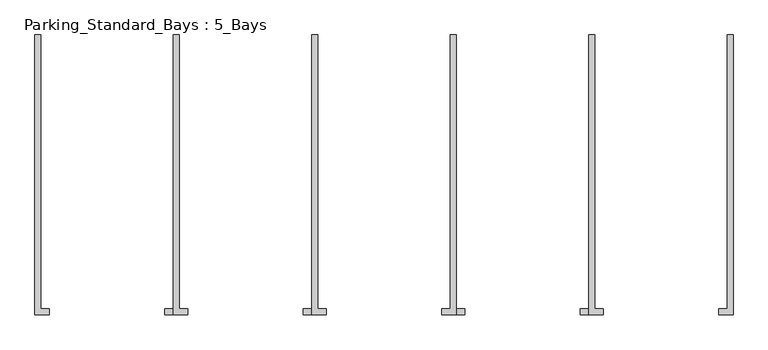
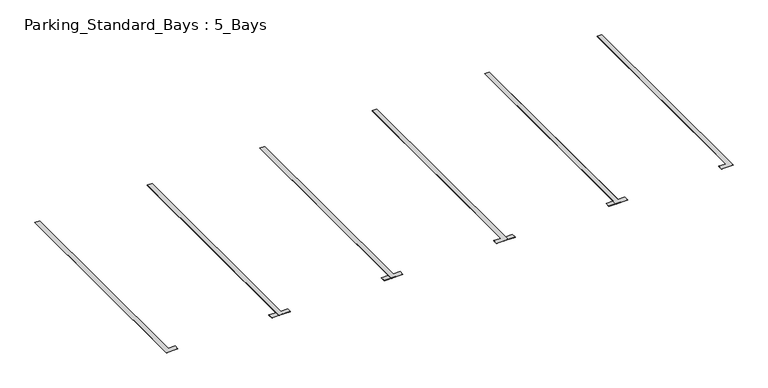
"""IFC4 building model written with IfcOpenShell, lengths in millimetres: proxy geometry, Parking_Standard_Bays : 5_Bays."""

import ifcopenshell
import ifcopenshell.guid

model = None  # the IFC model being written
_history = None  # IfcOwnerHistory: only IFC2X3 demands one
_inside = {}  # id of a spatial element -> (the spatial element, [elements in it])
_under = {}  # id of a project, library or spatial element -> (it, [spatial elements below it])
_declared = {}  # id of a project -> (the project, [libraries it declares])
_typed = {}  # id of a type object -> (the type object, [elements of that type])
_made_of = {}  # id of a material, layer set ... -> (it, [elements and type objects made of it])


def new_model(schema):
    """Start an empty IFC model of exactly this schema.

    Asked for "IFC4X3", IfcOpenShell would pick the latest addendum, in which some entities
    have other attributes; the version numbers below select the first issue.
    IFC2X3 requires an IfcOwnerHistory on every rooted entity: one is made here for all.
    """
    global model, _history
    if schema == "IFC4X3":
        model = ifcopenshell.file(schema_version=(4, 3, 0, 0))
    else:
        model = ifcopenshell.file(schema=schema)
    _inside.clear()
    _under.clear()
    _declared.clear()
    _typed.clear()
    _made_of.clear()
    _history = None
    if model.schema == "IFC2X3":
        org = make("IfcOrganization", Name="unknown")
        user = make(
            "IfcPersonAndOrganization",
            ThePerson=make("IfcPerson", FamilyName="unknown"),
            TheOrganization=org,
        )
        app = make(
            "IfcApplication",
            ApplicationDeveloper=org,
            Version="unknown",
            ApplicationFullName="unknown",
            ApplicationIdentifier="unknown",
        )
        _history = make(
            "IfcOwnerHistory",
            OwningUser=user,
            OwningApplication=app,
            ChangeAction="ADDED",
            CreationDate=0,
        )
    return model


def make(cls, **values):
    """One entity of the class cls with the attributes given. An attribute that is None is left unset."""
    return model.create_entity(
        cls, **{name: value for name, value in values.items() if value is not None}
    )


def rooted(cls, **values):
    """An entity with a GlobalId (a new one), such as an element, a storey or a relation."""
    return make(cls, GlobalId=ifcopenshell.guid.new(), OwnerHistory=_history, **values)


def si_unit(unit_type, name, prefix=None):
    """IfcSIUnit, for example si_unit("LENGTHUNIT", "METRE", prefix="MILLI")."""
    return make("IfcSIUnit", UnitType=unit_type, Prefix=prefix, Name=name)


def assignment(units):
    """IfcUnitAssignment: the units of a project."""
    return None if units is None else make("IfcUnitAssignment", Units=units)


def point(xyz):
    """IfcCartesianPoint."""
    return None if xyz is None else make("IfcCartesianPoint", Coordinates=xyz)


def direction(xyz):
    """IfcDirection."""
    return None if xyz is None else make("IfcDirection", DirectionRatios=xyz)


def frame(location, z_axis=None, x_axis=None):
    """IfcAxis2Placement3D, a coordinate frame: its origin and axes. An axis left out is left unset."""
    return make(
        "IfcAxis2Placement3D",
        Location=point(location),
        Axis=direction(z_axis),
        RefDirection=direction(x_axis),
    )


def origin():
    """The frame at (0, 0, 0) with its axes left unset."""
    return frame((0.0, 0.0, 0.0))


def origin_with_axes():
    """The frame at (0, 0, 0) with the z axis (0, 0, 1) and the x axis (1, 0, 0) written out."""
    return frame((0.0, 0.0, 0.0), z_axis=(0.0, 0.0, 1.0), x_axis=(1.0, 0.0, 0.0))


def place(relative_to, where):
    """IfcLocalPlacement: puts the frame where relative to a parent placement (None: the world)."""
    return make(
        "IfcLocalPlacement", PlacementRelTo=relative_to, RelativePlacement=where
    )


def context(
    kind, dimensions, precision=None, world=None, true_north=None, identifier=None
):
    """IfcGeometricRepresentationContext, for example the 3D "Model" context."""
    return make(
        "IfcGeometricRepresentationContext",
        ContextIdentifier=identifier,
        ContextType=kind,
        CoordinateSpaceDimension=dimensions,
        Precision=precision,
        WorldCoordinateSystem=world,
        TrueNorth=true_north,
    )


def project(units=None, contexts=None):
    """IfcProject with its units and contexts."""
    return rooted(
        "IfcProject",
        Name="project",
        RepresentationContexts=contexts,
        UnitsInContext=assignment(units),
    )


def spatial(cls, under=None, at=None, **own):
    """A site, building, storey or space (cls), placed at a placement, below another one or the project."""
    s = rooted(cls, ObjectPlacement=at, **own)
    if under is not None:
        _under.setdefault(under.id(), (under, []))[1].append(s)
    return s


def polyline(points):
    """IfcPolyline through the points."""
    return make("IfcPolyline", Points=[point(p) for p in points])


def outline(outer, holes=None, kind="AREA"):
    """IfcArbitraryClosedProfileDef: a profile drawn as a closed curve; with holes, ...WithVoids."""
    if holes is None:
        return make("IfcArbitraryClosedProfileDef", ProfileType=kind, OuterCurve=outer)
    return make(
        "IfcArbitraryProfileDefWithVoids",
        ProfileType=kind,
        OuterCurve=outer,
        InnerCurves=holes,
    )


def extrude(swept, where, along, depth):
    """IfcExtrudedAreaSolid: the profile swept, set in the frame where, extruded along a direction by depth."""
    return make(
        "IfcExtrudedAreaSolid",
        SweptArea=swept,
        Position=where,
        ExtrudedDirection=direction(along),
        Depth=depth,
    )


def shape(context_of_items, identifier, shape_type, items):
    """IfcShapeRepresentation: the items that make up one representation, for example the "Body"."""
    return make(
        "IfcShapeRepresentation",
        ContextOfItems=context_of_items,
        RepresentationIdentifier=identifier,
        RepresentationType=shape_type,
        Items=items,
    )


def source(mapping_origin, context_of_items, identifier, shape_type, items):
    """IfcRepresentationMap: a shape defined once, which mapped items show again and again."""
    return make(
        "IfcRepresentationMap",
        MappingOrigin=mapping_origin,
        MappedRepresentation=shape(context_of_items, identifier, shape_type, items),
    )


def transform(
    local_origin,
    x_axis=None,
    y_axis=None,
    z_axis=None,
    scale=None,
    scale2=None,
    scale3=None,
    uniform=True,
):
    """IfcCartesianTransformationOperator3D, or its non-uniform kind. x_axis, y_axis, z_axis: its Axis1, 2, 3."""
    if uniform:
        return make(
            "IfcCartesianTransformationOperator3D",
            Axis1=direction(x_axis),
            Axis2=direction(y_axis),
            LocalOrigin=point(local_origin),
            Scale=scale,
            Axis3=direction(z_axis),
        )
    return make(
        "IfcCartesianTransformationOperator3DnonUniform",
        Axis1=direction(x_axis),
        Axis2=direction(y_axis),
        LocalOrigin=point(local_origin),
        Scale=scale,
        Axis3=direction(z_axis),
        Scale2=scale2,
        Scale3=scale3,
    )


def mapped(mapping_source, mapping_target):
    """IfcMappedItem: shows the shape of a source again, moved by a transform."""
    return make(
        "IfcMappedItem", MappingSource=mapping_source, MappingTarget=mapping_target
    )


def made_of(thing, what):
    """Note that an element or type object is made of a material, layer set ...; save() writes the relation."""
    if what is not None:
        _made_of.setdefault(what.id(), (what, []))[1].append(thing)
    return thing


def element(
    cls,
    number,
    at=None,
    inside=None,
    cuts=None,
    type_object=None,
    material=None,
    context=None,
    identifier="Body",
    shape_type=None,
    held_by="IfcProductDefinitionShape",
    body=None,
    shapes=None,
    **own,
):
    """One element of the class cls, such as IfcWall. Its Tag is "e" and its number.

    at: its placement. inside: the storey or other place that contains it. cuts: it is an
    opening in that element (IfcRelVoidsElement). A single representation is given by context,
    identifier, shape_type and body (its items); several are given by shapes. held_by: the class
    of the entity that holds the representations. save() writes the other relations.
    """
    e = rooted(cls, Tag="e%d" % number, ObjectPlacement=at, **own)
    if body is not None:
        shapes = [shape(context, identifier, shape_type, body)]
    if shapes is not None:
        e.Representation = make(held_by, Representations=shapes)
    if inside is not None:
        _inside.setdefault(inside.id(), (inside, []))[1].append(e)
    if cuts is not None:
        rooted(
            "IfcRelVoidsElement", RelatingBuildingElement=cuts, RelatedOpeningElement=e
        )
    if type_object is not None:
        _typed.setdefault(type_object.id(), (type_object, []))[1].append(e)
    return made_of(e, material)


def aggregate(whole, parts):
    """IfcRelAggregates: a whole, such as a stair, and the parts it consists of."""
    return rooted("IfcRelAggregates", RelatingObject=whole, RelatedObjects=parts)


def save(model, path):
    """Write the relations noted so far, then the file.

    IfcRelAggregates (storeys below a building ...), IfcRelContainedInSpatialStructure (elements
    in a storey), IfcRelDefinesByType, IfcRelAssociatesMaterial and IfcRelDeclares: one each for
    every whole, place, type object, material and project.
    """
    for whole, parts in _under.values():
        aggregate(whole, parts)
    for where, things in _inside.values():
        rooted(
            "IfcRelContainedInSpatialStructure",
            RelatedElements=things,
            RelatingStructure=where,
        )
    for kind, things in _typed.values():
        rooted("IfcRelDefinesByType", RelatedObjects=things, RelatingType=kind)
    for what, things in _made_of.values():
        rooted("IfcRelAssociatesMaterial", RelatedObjects=things, RelatingMaterial=what)
    for by, libraries in _declared.values():
        rooted("IfcRelDeclares", RelatingContext=by, RelatedDefinitions=libraries)
    model.write(path)


def parking_standard_bays_5_bays_6c4ea7f3(model_context):
    return source(origin(), model_context, "Body", "SweptSolid", [
        extrude(outline(polyline([(11950.0, 0.0), (12050.0, 0.0), (12050.0, -4850.0), (11800.0, -4850.0), (11800.0, -4750.0), (11950.0, -4750.0), (11950.0, 0.0)])), origin_with_axes(), (0.0, 0.0, 1.0), 3.175),
        extrude(outline(polyline([(9550.0, 0.0), (9650.0, 0.0), (9650.0, -4750.0), (9800.0, -4750.0), (9800.0, -4850.0), (9550.0, -4850.0), (9550.0, 0.0)])), origin_with_axes(), (0.0, 0.0, 1.0), 3.175),
        extrude(outline(polyline([(7150.0, 0.0), (7250.0, 0.0), (7250.0, -4850.0), (7000.0, -4850.0), (7000.0, -4750.0), (7150.0, -4750.0), (7150.0, 0.0)])), origin_with_axes(), (0.0, 0.0, 1.0), 3.175),
        extrude(outline(polyline([(4750.0, 0.0), (4850.0, 0.0), (4850.0, -4750.0), (5000.0, -4750.0), (5000.0, -4850.0), (4750.0, -4850.0), (4750.0, 0.0)])), origin_with_axes(), (0.0, 0.0, 1.0), 3.175),
        extrude(outline(polyline([(4750.0, 0.0), (4850.0, 0.0), (4850.0, -4850.0), (4600.0, -4850.0), (4600.0, -4750.0), (4750.0, -4750.0), (4750.0, 0.0)])), origin_with_axes(), (0.0, 0.0, 1.0), 3.175),
        extrude(outline(polyline([(2350.0, 0.0), (2450.0, 0.0), (2450.0, -4750.0), (2600.0, -4750.0), (2600.0, -4850.0), (2350.0, -4850.0), (2350.0, 0.0)])), origin_with_axes(), (0.0, 0.0, 1.0), 3.175),
        extrude(outline(polyline([(9550.0, 0.0), (9650.0, 0.0), (9650.0, -4850.0), (9400.0, -4850.0), (9400.0, -4750.0), (9550.0, -4750.0), (9550.0, 0.0)])), origin_with_axes(), (0.0, 0.0, 1.0), 3.175),
        extrude(outline(polyline([(7150.0, 0.0), (7250.0, 0.0), (7250.0, -4750.0), (7400.0, -4750.0), (7400.0, -4850.0), (7150.0, -4850.0), (7150.0, 0.0)])), origin_with_axes(), (0.0, 0.0, 1.0), 3.175),
        extrude(outline(polyline([(2350.0, 0.0), (2450.0, 0.0), (2450.0, -4850.0), (2200.0, -4850.0), (2200.0, -4750.0), (2350.0, -4750.0), (2350.0, 0.0)])), origin_with_axes(), (0.0, 0.0, 1.0), 3.175),
        extrude(outline(polyline([(-50.0, 0.0), (50.0, 0.0), (50.0, -4750.0), (200.0, -4750.0), (200.0, -4850.0), (-50.0, -4850.0), (-50.0, 0.0)])), origin_with_axes(), (0.0, 0.0, 1.0), 3.175),
    ])


if __name__ == "__main__":
    model = new_model("IFC4")
    model_context = context("Model", 3, world=origin())
    ifc_project = project(units=[si_unit("LENGTHUNIT", "METRE", prefix="MILLI")], contexts=[model_context])
    site = spatial("IfcSite", under=ifc_project)
    building = spatial("IfcBuilding", under=site)
    placement = place(None, origin())
    parking_standard_bays_5_bays_shape = parking_standard_bays_5_bays_6c4ea7f3(model_context)
    element("IfcBuildingElementProxy", 1, Name="Parking_Standard_Bays : 5_Bays", ObjectType="Parking_Standard_Bays : 5_Bays", at=placement, inside=building, context=model_context, shape_type="MappedRepresentation", body=[
        mapped(parking_standard_bays_5_bays_shape, transform((0.0, 0.0, 0.0), x_axis=(1.0, 0.0, 0.0), y_axis=(0.0, 1.0, 0.0), z_axis=(0.0, 0.0, 1.0))),
    ])
    save(model, "model.ifc")

# Revit data of these elements
# Type "Parking_Standard_Bays : 5_Bays"
#   Keynote = "Q22/185"
#   Length [instance default] = 14400 mm
#   Bay Width = 2400 mm
#   Bay Length = 4800 mm
#   No of Bays in Array [instance default] = 5
#   No of Bays [instance default] = 6
#   Material - White Lining = Paint - White Lining
# Element 1 (IfcBuildingElementProxy, "Parking_Standard_Bays : 5_Bays")
#   Length = 12000 mm
#   No of Bays in Array = 4
#   No of Bays = 5
#   Materials on its faces: "Paint - White Lining"
# Materials
#   "Paint - White Lining": class "Paint", colour RGB 239 247 247, transparency 0
